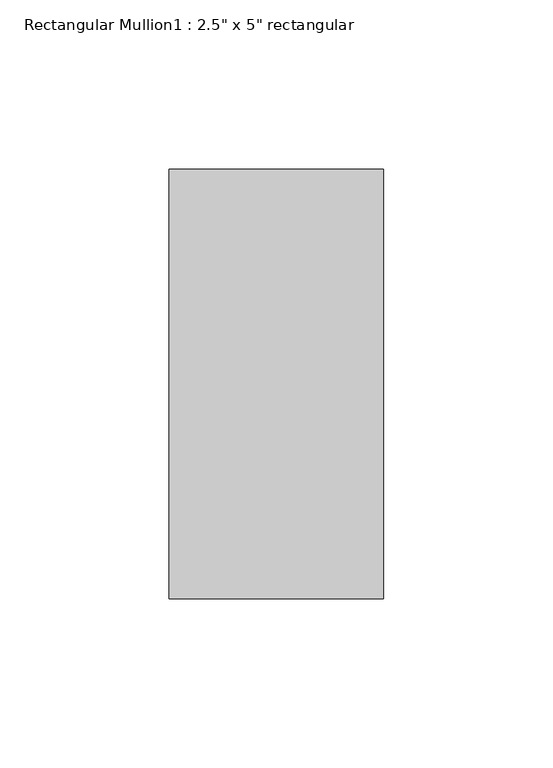
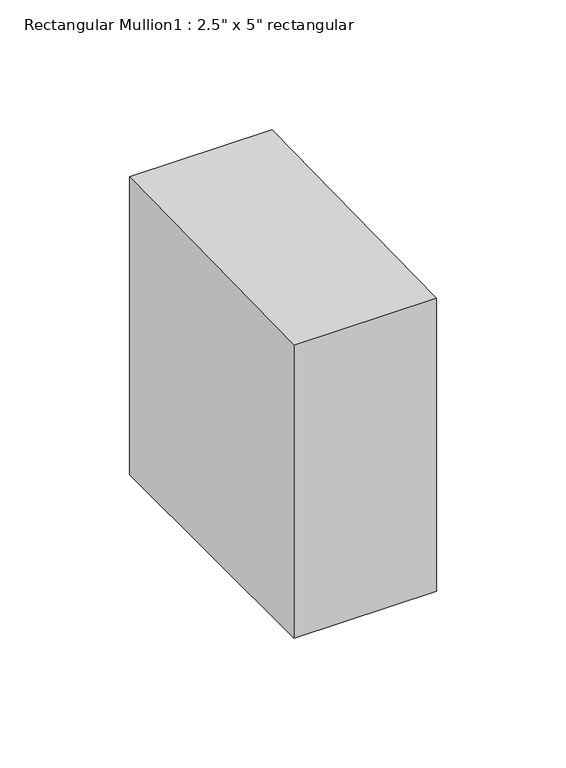
"""IFC4 building model written with IfcOpenShell, lengths in millimetres: member geometry."""

from ifc_helpers import new_model, si_unit, frame, origin, place, context, project, spatial, polyline, outline, extrude, source, transform, mapped, element, save


def member_b1809f7d(model_context):
    return source(origin(), model_context, "Body", "SweptSolid", [
        extrude(outline(polyline([(-63.5, -1.2595978), (63.5, 1.1843556), (63.5, -139.2998379), (-63.5, -139.2998379), (-63.5, -1.2595978)])), frame((-63.5, 0.0, 0.0), z_axis=(1.0, 0.0, 0.0), x_axis=(0.0, 1.0, 0.0)), (0.0, 0.0, 1.0), 63.5),
    ])


if __name__ == "__main__":
    model = new_model("IFC4")
    model_context = context("Model", 3, world=origin())
    ifc_project = project(units=[si_unit("LENGTHUNIT", "METRE", prefix="MILLI")], contexts=[model_context])
    site = spatial("IfcSite", under=ifc_project)
    building = spatial("IfcBuilding", under=site)
    placement = place(None, origin())
    member_shape = member_b1809f7d(model_context)
    element("IfcMember", 1, ObjectType="Rectangular Mullion1 : 2.5\" x 5\" rectangular", at=placement, inside=building, context=model_context, shape_type="MappedRepresentation", body=[
        mapped(member_shape, transform((0.0, 0.0, 0.0), x_axis=(1.0, 0.0, 0.0), y_axis=(0.0, 1.0, 0.0), z_axis=(0.0, 0.0, 1.0))),
    ])
    save(model, "model.ifc")

# Revit data of these elements
# Type "Rectangular Mullion1 : 2.5\" x 5\" rectangular"
#   built-in parameter 1007304 = 0.416667 (stored number, unit not read)
#   built-in parameter 1007301 = 0.104167 (stored number, unit not read)
#   built-in parameter 1007300 = 0.104167 (stored number, unit not read)
# Element 1 (IfcMember, "Rectangular Mullion1 : 2.5\" x 5\" rectangular")
#   Materials on its faces: "support-frame"
# Materials
#   "support-frame": class "Unassigned", colour RGB 233 233 233, transparency 0, Cost = 0
